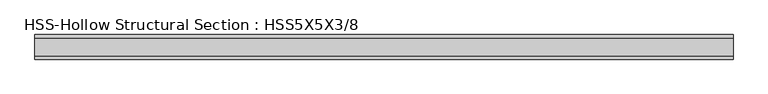
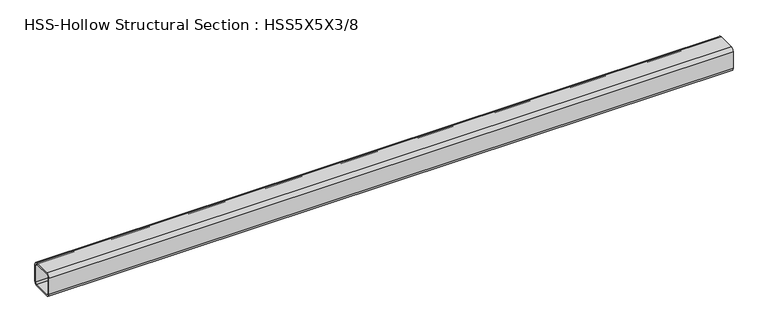
"""IFC4 building model written with IfcOpenShell, lengths in millimetres: member geometry, HSS-Hollow Structural Section : HSS5X5X3/8."""

from ifc_helpers import new_model, si_unit, point, frame, frame_2d, origin, place, context, project, spatial, polyline, circle_curve, trimmed, segment, composite_curve, outline, extrude, source, transform, mapped, element, save


def hss_hollow_structural_section_hss5x5x3_8_44a837d7(model_context):
    return source(origin(), model_context, "Body", "SweptSolid", [
        extrude(outline(composite_curve([segment(polyline([(63.5, 45.7708), (63.5, -45.7708)]), True, "CONTINUOUS"), segment(trimmed(circle_curve(frame_2d((45.7708, -45.7708)), 17.7292), [point((63.5, -45.7708))], [point((45.7708, -63.5))], False, "CARTESIAN"), True, "CONTINUOUS"), segment(polyline([(45.7708, -63.5), (-45.7708, -63.5)]), True, "CONTINUOUS"), segment(trimmed(circle_curve(frame_2d((-45.7708, -45.7708)), 17.7292), [point((-45.7708, -63.5))], [point((-63.5, -45.7708))], False, "CARTESIAN"), True, "CONTINUOUS"), segment(polyline([(-63.5, -45.7708), (-63.5, 45.7708)]), True, "CONTINUOUS"), segment(trimmed(circle_curve(frame_2d((-45.7708, 45.7708)), 17.7292), [point((-63.5, 45.7708))], [point((-45.7708, 63.5))], False, "CARTESIAN"), True, "CONTINUOUS"), segment(polyline([(-45.7708, 63.5), (45.7708, 63.5)]), True, "CONTINUOUS"), segment(trimmed(circle_curve(frame_2d((45.7708, 45.7708)), 17.7292), [point((45.7708, 63.5))], [point((63.5, 45.7708))], False, "CARTESIAN"), True, "CONTINUOUS")], self_intersect=False), holes=[composite_curve([segment(trimmed(circle_curve(frame_2d((-45.7708, 45.7708)), 8.8646), [point((-45.7708, 54.6354))], [point((-54.6354, 45.7708))], True, "CARTESIAN"), True, "CONTINUOUS"), segment(polyline([(-54.6354, 45.7708), (-54.6354, -45.7708)]), True, "CONTINUOUS"), segment(trimmed(circle_curve(frame_2d((-45.7708, -45.7708)), 8.8646), [point((-54.6354, -45.7708))], [point((-45.7708, -54.6354))], True, "CARTESIAN"), True, "CONTINUOUS"), segment(polyline([(-45.7708, -54.6354), (45.7708, -54.6354)]), True, "CONTINUOUS"), segment(trimmed(circle_curve(frame_2d((45.7708, -45.7708)), 8.8646), [point((45.7708, -54.6354))], [point((54.6354, -45.7708))], True, "CARTESIAN"), True, "CONTINUOUS"), segment(polyline([(54.6354, -45.7708), (54.6354, 45.7708)]), True, "CONTINUOUS"), segment(trimmed(circle_curve(frame_2d((45.7708, 45.7708)), 8.8646), [point((54.6354, 45.7708))], [point((45.7708, 54.6354))], True, "CARTESIAN"), True, "CONTINUOUS"), segment(polyline([(45.7708, 54.6354), (-45.7708, 54.6354)]), True, "CONTINUOUS")], self_intersect=False)]), frame((-1802.7532185, 0.0, 0.0), z_axis=(1.0, 0.0, 0.0), x_axis=(0.0, 1.0, 0.0)), (0.0, 0.0, 1.0), 3605.506437),
    ])


if __name__ == "__main__":
    model = new_model("IFC4")
    model_context = context("Model", 3, world=origin())
    ifc_project = project(units=[si_unit("LENGTHUNIT", "METRE", prefix="MILLI")], contexts=[model_context])
    site = spatial("IfcSite", under=ifc_project)
    building = spatial("IfcBuilding", under=site)
    placement = place(None, origin())
    hss_hollow_structural_section_hss5x5x3_8_shape = hss_hollow_structural_section_hss5x5x3_8_44a837d7(model_context)
    element("IfcMember", 1, ObjectType="HSS-Hollow Structural Section : HSS5X5X3/8", at=placement, inside=building, context=model_context, shape_type="MappedRepresentation", body=[
        mapped(hss_hollow_structural_section_hss5x5x3_8_shape, transform((0.0, 0.0, 0.0), x_axis=(1.0, 0.0, 0.0), y_axis=(0.0, 1.0, 0.0), z_axis=(0.0, 0.0, 1.0))),
    ])
    save(model, "model.ifc")

# Revit data of these elements
# Type "HSS-Hollow Structural Section : HSS5X5X3/8"
#   Assembly Code = "B10"
#   Shape = "Square"
#   W = 22.3
#   Ht = 0' - 5"
#   Length [instance default] = 5' - 0"
#   b = 0' - 5"
#   kr = 0' - 0.698"
#   t = 0' - 0.349"
#   A = 0.0429167 SF
#   Structural Material [instance default] = Steel ASTM A500, Grade B, Rectangular and Square
# Element 1 (IfcMember, "HSS-Hollow Structural Section : HSS5X5X3/8")
#   Materials on its faces: "Steel ASTM A500, Grade B, Rectangular and Square"
# Materials
#   "Steel ASTM A500, Grade B, Rectangular and Square": class "Metal", colour RGB 199 199 199, transparency 0, Description = "Carbon steel", Cost = 0
